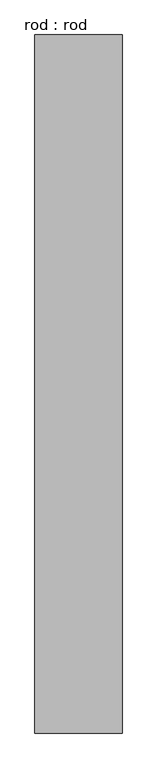
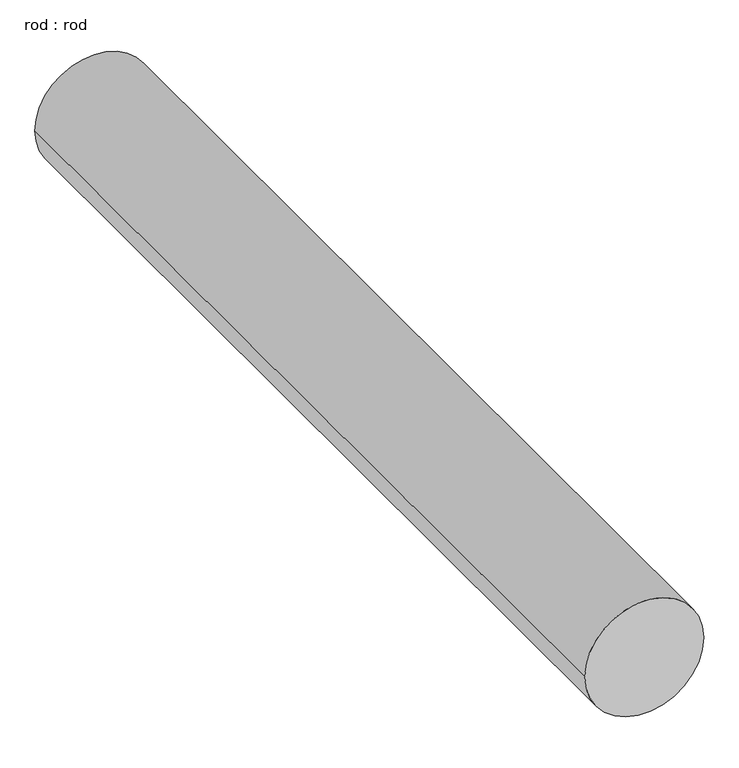
"""IFC4 building model written with IfcOpenShell, lengths in millimetres: proxy geometry, rod : rod."""

from ifc_helpers import new_model, si_unit, point, frame, frame_2d, origin, place, context, project, spatial, circle_curve, trimmed, segment, composite_curve, outline, extrude, source, transform, mapped, element, save


def rod_rod_ad616e14(model_context):
    return source(origin(), model_context, "Body", "SweptSolid", [
        extrude(outline(composite_curve([segment(trimmed(circle_curve(frame_2d((0.0108462, 0.0)), 200.0), [point((0.0108462, 200.0))], [point((0.0108462, -200.0))], False, "CARTESIAN"), True, "CONTINUOUS"), segment(trimmed(circle_curve(frame_2d((0.0108462, 0.0)), 200.0), [point((0.0108462, -200.0))], [point((0.0108462, 200.0))], False, "CARTESIAN"), True, "CONTINUOUS")], self_intersect=False)), frame((0.0, 2490.9429011, 0.0), z_axis=(0.0, 1.0, 0.0), x_axis=(0.0, 0.0, 1.0)), (0.0, 0.0, 1.0), 3203.5714286),
    ])


if __name__ == "__main__":
    model = new_model("IFC4")
    model_context = context("Model", 3, world=origin())
    ifc_project = project(units=[si_unit("LENGTHUNIT", "METRE", prefix="MILLI")], contexts=[model_context])
    site = spatial("IfcSite", under=ifc_project)
    building = spatial("IfcBuilding", under=site)
    placement = place(None, origin())
    rod_rod_shape = rod_rod_ad616e14(model_context)
    element("IfcBuildingElementProxy", 1, Name="rod : rod", ObjectType="rod : rod", at=placement, inside=building, context=model_context, shape_type="MappedRepresentation", body=[
        mapped(rod_rod_shape, transform((0.0, 0.0, 0.0), x_axis=(1.0, 0.0, 0.0), y_axis=(0.0, 1.0, 0.0), z_axis=(0.0, 0.0, 1.0))),
    ])
    save(model, "model.ifc")

# Revit data of these elements
# Type "rod : rod"
#   Default Elevation = 0
